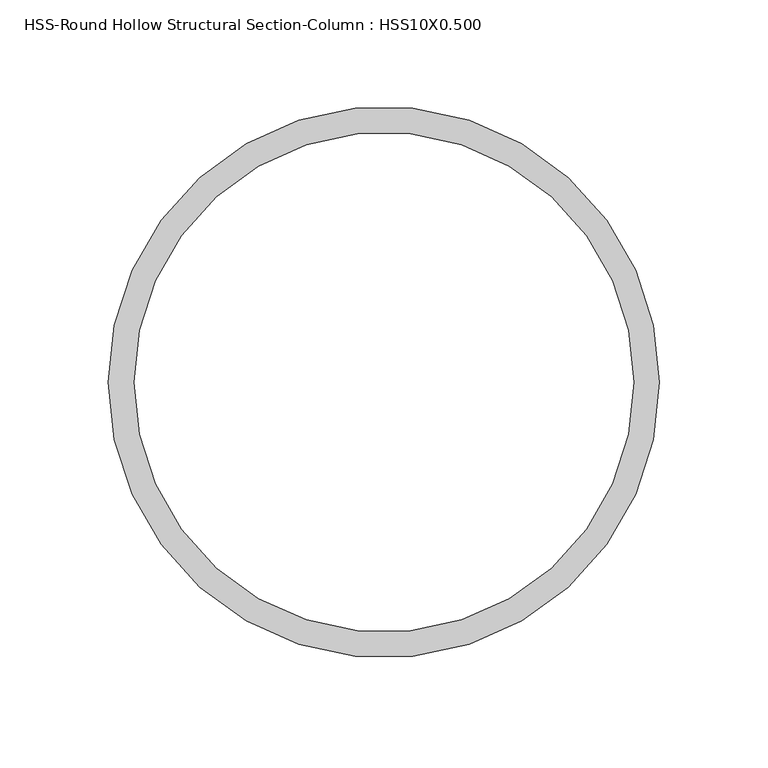
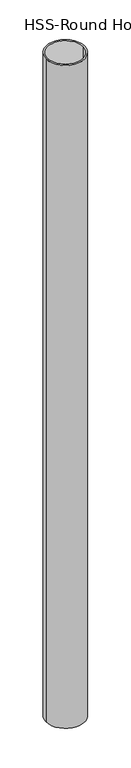
"""IFC4 building model written with IfcOpenShell, lengths in millimetres: column geometry, HSS-Round Hollow Structural Section-Column : HSS10X0.500."""

from ifc_helpers import new_model, si_unit, point, frame, origin, origin_2d, place, context, project, spatial, circle_curve, trimmed, segment, composite_curve, outline, extrude, source, transform, mapped, element, save


def hss_round_hollow_structural_section_column_hss10x0_500_8cda41c0(model_context):
    return source(origin(), model_context, "Body", "SweptSolid", [
        extrude(outline(composite_curve([segment(trimmed(circle_curve(origin_2d(), 127.0), [point((-127.0, 0.0))], [point((127.0, 0.0))], False, "CARTESIAN"), True, "CONTINUOUS"), segment(trimmed(circle_curve(origin_2d(), 127.0), [point((127.0, 0.0))], [point((-127.0, 0.0))], False, "CARTESIAN"), True, "CONTINUOUS")], self_intersect=False), holes=[composite_curve([segment(trimmed(circle_curve(origin_2d(), 115.189), [point((-115.189, 0.0))], [point((115.189, 0.0))], True, "CARTESIAN"), True, "CONTINUOUS"), segment(trimmed(circle_curve(origin_2d(), 115.189), [point((115.189, 0.0))], [point((-115.189, 0.0))], True, "CARTESIAN"), True, "CONTINUOUS")], self_intersect=False)]), frame((0.0, 0.0, 10541.0), z_axis=(0.0, 0.0, 1.0), x_axis=(1.0, 0.0, 0.0)), (0.0, 0.0, 1.0), 4572.0),
    ])


if __name__ == "__main__":
    model = new_model("IFC4")
    model_context = context("Model", 3, world=origin())
    ifc_project = project(units=[si_unit("LENGTHUNIT", "METRE", prefix="MILLI")], contexts=[model_context])
    site = spatial("IfcSite", under=ifc_project)
    building = spatial("IfcBuilding", under=site)
    placement = place(None, origin())
    hss_round_hollow_structural_section_column_hss10x0_500_shape = hss_round_hollow_structural_section_column_hss10x0_500_8cda41c0(model_context)
    element("IfcColumn", 1, ObjectType="HSS-Round Hollow Structural Section-Column : HSS10X0.500", at=placement, inside=building, context=model_context, shape_type="MappedRepresentation", body=[
        mapped(hss_round_hollow_structural_section_column_hss10x0_500_shape, transform((0.0, 0.0, 0.0), x_axis=(1.0, 0.0, 0.0), y_axis=(0.0, 1.0, 0.0), z_axis=(0.0, 0.0, 1.0))),
    ])
    save(model, "model.ifc")

# Revit data of these elements
# Type "HSS-Round Hollow Structural Section-Column : HSS10X0.500"
#   Assembly Code = "B10"
#   W = 50.8
#   OD = 0' - 10"
#   t = 0' - 0.465"
#   A = 0.0965278 SF
#   Column Material [instance default] = Metal - Steel - ASTM A53
# Element 1 (IfcColumn, "HSS-Round Hollow Structural Section-Column : HSS10X0.500")
#   Materials on its faces: "Metal - Steel - ASTM A53"
# Materials
#   "Metal - Steel - ASTM A53": class "Metal", colour RGB 128 0 0, transparency 0
